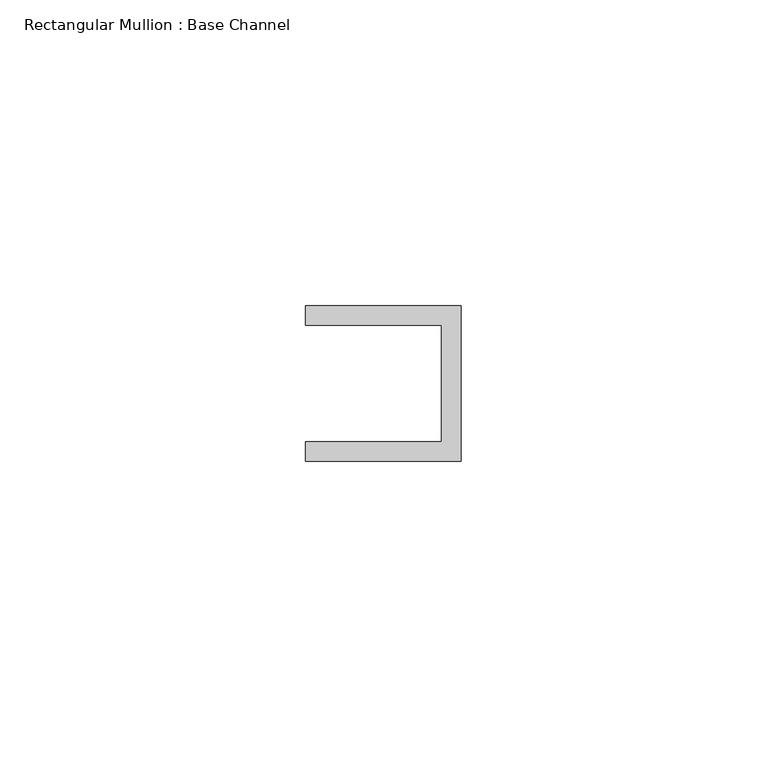
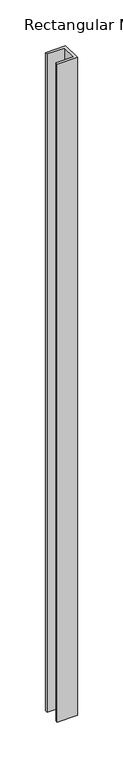
"""IFC4 building model written with IfcOpenShell, lengths in millimetres: member geometry, Rectangular Mullion : Base Channel."""

from ifc_helpers import new_model, si_unit, frame, origin, place, context, project, spatial, polyline, outline, extrude, source, transform, mapped, element, save


def rectangular_mullion_base_channel_83215bdc(model_context):
    return source(origin(), model_context, "Body", "SweptSolid", [
        extrude(outline(polyline([(0.0, 12.7), (0.0, -12.7), (-25.4, -12.7), (-25.4, -9.525), (-3.175, -9.525), (-3.175, 9.525), (-25.4, 9.525), (-25.4, 12.7), (0.0, 12.7)])), frame((0.0, 0.0, -876.6175002), z_axis=(0.0, 0.0, 1.0), x_axis=(1.0, 0.0, 0.0)), (0.0, 0.0, 1.0), 876.6175002),
    ])


if __name__ == "__main__":
    model = new_model("IFC4")
    model_context = context("Model", 3, world=origin())
    ifc_project = project(units=[si_unit("LENGTHUNIT", "METRE", prefix="MILLI")], contexts=[model_context])
    site = spatial("IfcSite", under=ifc_project)
    building = spatial("IfcBuilding", under=site)
    placement = place(None, origin())
    rectangular_mullion_base_channel_shape = rectangular_mullion_base_channel_83215bdc(model_context)
    element("IfcMember", 1, ObjectType="Rectangular Mullion : Base Channel", at=placement, inside=building, context=model_context, shape_type="MappedRepresentation", body=[
        mapped(rectangular_mullion_base_channel_shape, transform((0.0, 0.0, 0.0), x_axis=(1.0, 0.0, 0.0), y_axis=(0.0, 1.0, 0.0), z_axis=(0.0, 0.0, 1.0))),
    ])
    save(model, "model.ifc")

# Revit data of these elements
# Type "Rectangular Mullion : Base Channel"
#   built-in parameter 1007322 = 0.0833333 (stored number, unit not read)
#   built-in parameter 1007321 = 0.0416667 (stored number, unit not read)
#   built-in parameter 1007320 = -0.03125 (stored number, unit not read)
# Element 1 (IfcMember, "Rectangular Mullion : Base Channel")
#   Materials on its faces: "ALUM"
# Materials
#   "ALUM": class "Generic", colour RGB 157 157 157, transparency 0, Cost = 0
